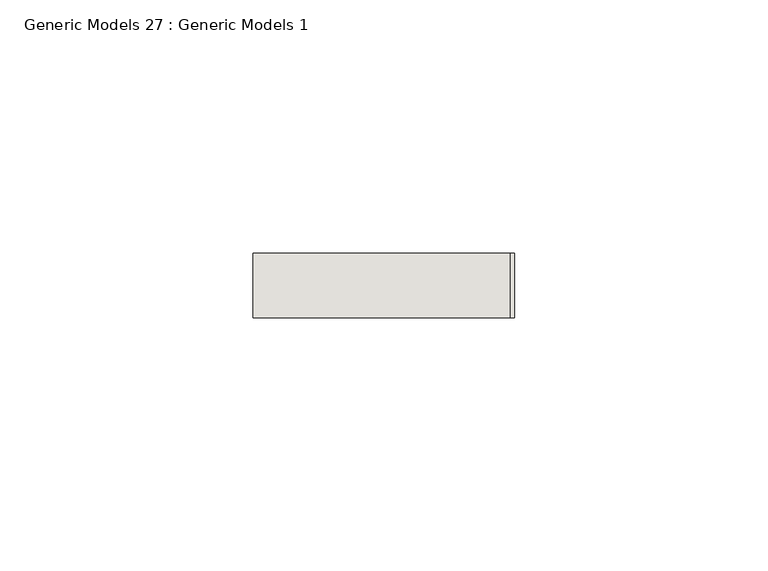
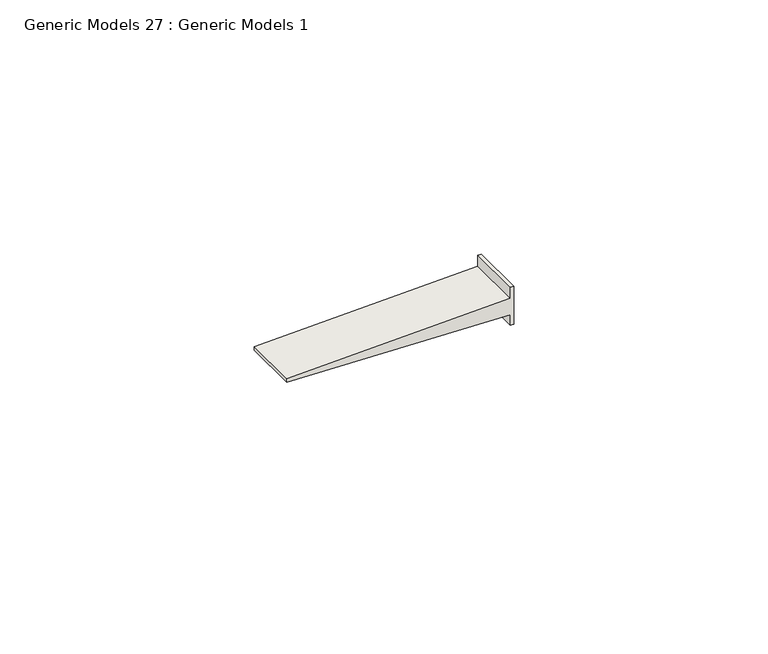
"""IFC4 building model written with IfcOpenShell, lengths in millimetres: wall geometry, Generic Models 27 : Generic Models 1."""

from ifc_helpers import new_model, si_unit, frame, origin, place, context, project, spatial, polyline, outline, extrude, source, transform, mapped, element, save


def generic_models_27_generic_models_1_e5767157(model_context):
    return source(origin(), model_context, "Body", "SweptSolid", [
        extrude(outline(polyline([(2409.6091, 49800.66875), (2409.6091, 49799.875), (2407.0592364, 49799.875), (2405.4618473, 49749.075), (2404.6631527, 49749.075), (2403.0657636, 49799.875), (2400.5159, 49799.875), (2400.5159, 49800.66875), (2409.6091, 49800.66875)])), frame((0.0, 565.15, 0.0), z_axis=(0.0, 1.0, 0.0), x_axis=(0.0, 0.0, 1.0)), (0.0, 0.0, 1.0), 12.7),
    ])


if __name__ == "__main__":
    model = new_model("IFC4")
    model_context = context("Model", 3, world=origin())
    ifc_project = project(units=[si_unit("LENGTHUNIT", "METRE", prefix="MILLI")], contexts=[model_context])
    site = spatial("IfcSite", under=ifc_project)
    building = spatial("IfcBuilding", under=site)
    placement = place(None, origin())
    generic_models_27_generic_models_1_shape = generic_models_27_generic_models_1_e5767157(model_context)
    element("IfcWall", 1, ObjectType="Generic Models 27 : Generic Models 1", at=placement, inside=building, context=model_context, shape_type="MappedRepresentation", body=[
        mapped(generic_models_27_generic_models_1_shape, transform((0.0, 0.0, 0.0), x_axis=(1.0, 0.0, 0.0), y_axis=(0.0, 1.0, 0.0), z_axis=(0.0, 0.0, 1.0))),
    ])
    save(model, "model.ifc")

# Revit data of these elements
# Element 1 (IfcWall, "Generic Models 27 : Generic Models 1")
#   Materials on its faces: "ATTACH GYPSUM BOARD TO STUDS AND NOT TO TOP TRACK"
# Materials
#   "ATTACH GYPSUM BOARD TO STUDS AND NOT TO TOP TRACK": class "Generic", colour RGB 48 48 48, transparency 0, Cost = 0
